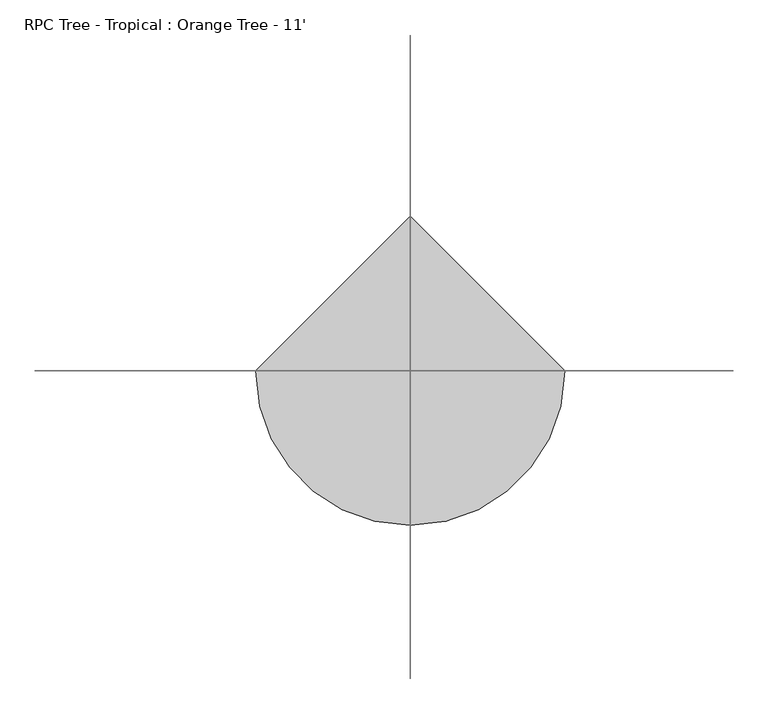
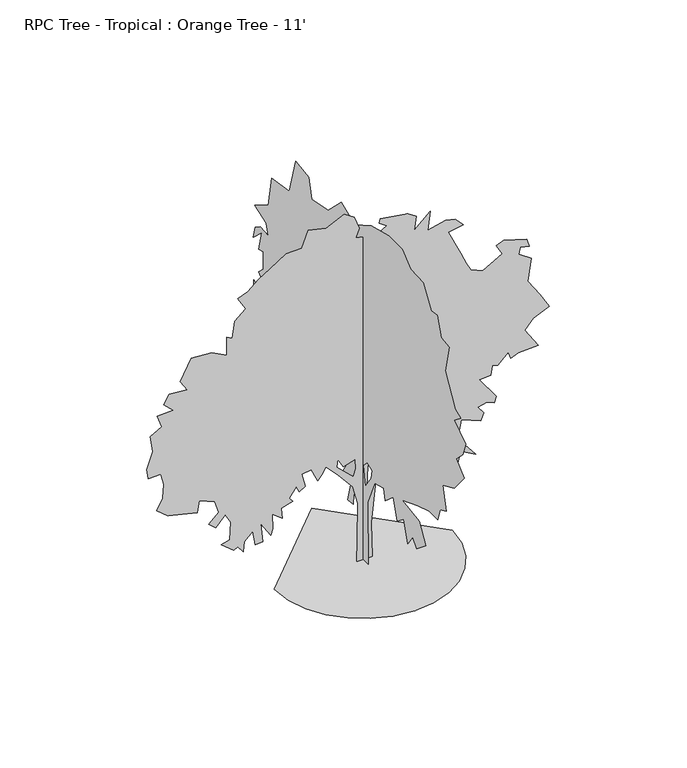
"""IFC4 building model written with IfcOpenShell, lengths in millimetres: geographic element geometry, RPC Tree - Tropical : Orange Tree - 11'."""

import ifcopenshell
import ifcopenshell.guid

model = None  # the IFC model being written
_history = None  # IfcOwnerHistory: only IFC2X3 demands one
_inside = {}  # id of a spatial element -> (the spatial element, [elements in it])
_under = {}  # id of a project, library or spatial element -> (it, [spatial elements below it])
_declared = {}  # id of a project -> (the project, [libraries it declares])
_typed = {}  # id of a type object -> (the type object, [elements of that type])
_made_of = {}  # id of a material, layer set ... -> (it, [elements and type objects made of it])


def new_model(schema):
    """Start an empty IFC model of exactly this schema.

    Asked for "IFC4X3", IfcOpenShell would pick the latest addendum, in which some entities
    have other attributes; the version numbers below select the first issue.
    IFC2X3 requires an IfcOwnerHistory on every rooted entity: one is made here for all.
    """
    global model, _history
    if schema == "IFC4X3":
        model = ifcopenshell.file(schema_version=(4, 3, 0, 0))
    else:
        model = ifcopenshell.file(schema=schema)
    _inside.clear()
    _under.clear()
    _declared.clear()
    _typed.clear()
    _made_of.clear()
    _history = None
    if model.schema == "IFC2X3":
        org = make("IfcOrganization", Name="unknown")
        user = make(
            "IfcPersonAndOrganization",
            ThePerson=make("IfcPerson", FamilyName="unknown"),
            TheOrganization=org,
        )
        app = make(
            "IfcApplication",
            ApplicationDeveloper=org,
            Version="unknown",
            ApplicationFullName="unknown",
            ApplicationIdentifier="unknown",
        )
        _history = make(
            "IfcOwnerHistory",
            OwningUser=user,
            OwningApplication=app,
            ChangeAction="ADDED",
            CreationDate=0,
        )
    return model


def make(cls, **values):
    """One entity of the class cls with the attributes given. An attribute that is None is left unset."""
    return model.create_entity(
        cls, **{name: value for name, value in values.items() if value is not None}
    )


def rooted(cls, **values):
    """An entity with a GlobalId (a new one), such as an element, a storey or a relation."""
    return make(cls, GlobalId=ifcopenshell.guid.new(), OwnerHistory=_history, **values)


def si_unit(unit_type, name, prefix=None):
    """IfcSIUnit, for example si_unit("LENGTHUNIT", "METRE", prefix="MILLI")."""
    return make("IfcSIUnit", UnitType=unit_type, Prefix=prefix, Name=name)


def assignment(units):
    """IfcUnitAssignment: the units of a project."""
    return None if units is None else make("IfcUnitAssignment", Units=units)


def point(xyz):
    """IfcCartesianPoint."""
    return None if xyz is None else make("IfcCartesianPoint", Coordinates=xyz)


def direction(xyz):
    """IfcDirection."""
    return None if xyz is None else make("IfcDirection", DirectionRatios=xyz)


def frame(location, z_axis=None, x_axis=None):
    """IfcAxis2Placement3D, a coordinate frame: its origin and axes. An axis left out is left unset."""
    return make(
        "IfcAxis2Placement3D",
        Location=point(location),
        Axis=direction(z_axis),
        RefDirection=direction(x_axis),
    )


def origin():
    """The frame at (0, 0, 0) with its axes left unset."""
    return frame((0.0, 0.0, 0.0))


def place(relative_to, where):
    """IfcLocalPlacement: puts the frame where relative to a parent placement (None: the world)."""
    return make(
        "IfcLocalPlacement", PlacementRelTo=relative_to, RelativePlacement=where
    )


def context(
    kind, dimensions, precision=None, world=None, true_north=None, identifier=None
):
    """IfcGeometricRepresentationContext, for example the 3D "Model" context."""
    return make(
        "IfcGeometricRepresentationContext",
        ContextIdentifier=identifier,
        ContextType=kind,
        CoordinateSpaceDimension=dimensions,
        Precision=precision,
        WorldCoordinateSystem=world,
        TrueNorth=true_north,
    )


def project(units=None, contexts=None):
    """IfcProject with its units and contexts."""
    return rooted(
        "IfcProject",
        Name="project",
        RepresentationContexts=contexts,
        UnitsInContext=assignment(units),
    )


def spatial(cls, under=None, at=None, **own):
    """A site, building, storey or space (cls), placed at a placement, below another one or the project."""
    s = rooted(cls, ObjectPlacement=at, **own)
    if under is not None:
        _under.setdefault(under.id(), (under, []))[1].append(s)
    return s


def point_list(points):
    """IfcCartesianPointList2D or 3D."""
    cls = (
        "IfcCartesianPointList2D" if len(points[0]) == 2 else "IfcCartesianPointList3D"
    )
    return make(cls, CoordList=points)


def triangles(points, corners, closed=None, point_numbers=None):
    """IfcTriangulatedFaceSet: each triangle names its three corners, points numbered from 1."""
    return make(
        "IfcTriangulatedFaceSet",
        Coordinates=point_list(points),
        Closed=closed,
        CoordIndex=corners,
        PnIndex=point_numbers,
    )


def shape(context_of_items, identifier, shape_type, items):
    """IfcShapeRepresentation: the items that make up one representation, for example the "Body"."""
    return make(
        "IfcShapeRepresentation",
        ContextOfItems=context_of_items,
        RepresentationIdentifier=identifier,
        RepresentationType=shape_type,
        Items=items,
    )


def source(mapping_origin, context_of_items, identifier, shape_type, items):
    """IfcRepresentationMap: a shape defined once, which mapped items show again and again."""
    return make(
        "IfcRepresentationMap",
        MappingOrigin=mapping_origin,
        MappedRepresentation=shape(context_of_items, identifier, shape_type, items),
    )


def transform(
    local_origin,
    x_axis=None,
    y_axis=None,
    z_axis=None,
    scale=None,
    scale2=None,
    scale3=None,
    uniform=True,
):
    """IfcCartesianTransformationOperator3D, or its non-uniform kind. x_axis, y_axis, z_axis: its Axis1, 2, 3."""
    if uniform:
        return make(
            "IfcCartesianTransformationOperator3D",
            Axis1=direction(x_axis),
            Axis2=direction(y_axis),
            LocalOrigin=point(local_origin),
            Scale=scale,
            Axis3=direction(z_axis),
        )
    return make(
        "IfcCartesianTransformationOperator3DnonUniform",
        Axis1=direction(x_axis),
        Axis2=direction(y_axis),
        LocalOrigin=point(local_origin),
        Scale=scale,
        Axis3=direction(z_axis),
        Scale2=scale2,
        Scale3=scale3,
    )


def mapped(mapping_source, mapping_target):
    """IfcMappedItem: shows the shape of a source again, moved by a transform."""
    return make(
        "IfcMappedItem", MappingSource=mapping_source, MappingTarget=mapping_target
    )


def made_of(thing, what):
    """Note that an element or type object is made of a material, layer set ...; save() writes the relation."""
    if what is not None:
        _made_of.setdefault(what.id(), (what, []))[1].append(thing)
    return thing


def element(
    cls,
    number,
    at=None,
    inside=None,
    cuts=None,
    type_object=None,
    material=None,
    context=None,
    identifier="Body",
    shape_type=None,
    held_by="IfcProductDefinitionShape",
    body=None,
    shapes=None,
    **own,
):
    """One element of the class cls, such as IfcWall. Its Tag is "e" and its number.

    at: its placement. inside: the storey or other place that contains it. cuts: it is an
    opening in that element (IfcRelVoidsElement). A single representation is given by context,
    identifier, shape_type and body (its items); several are given by shapes. held_by: the class
    of the entity that holds the representations. save() writes the other relations.
    """
    e = rooted(cls, Tag="e%d" % number, ObjectPlacement=at, **own)
    if body is not None:
        shapes = [shape(context, identifier, shape_type, body)]
    if shapes is not None:
        e.Representation = make(held_by, Representations=shapes)
    if inside is not None:
        _inside.setdefault(inside.id(), (inside, []))[1].append(e)
    if cuts is not None:
        rooted(
            "IfcRelVoidsElement", RelatingBuildingElement=cuts, RelatedOpeningElement=e
        )
    if type_object is not None:
        _typed.setdefault(type_object.id(), (type_object, []))[1].append(e)
    return made_of(e, material)


def aggregate(whole, parts):
    """IfcRelAggregates: a whole, such as a stair, and the parts it consists of."""
    return rooted("IfcRelAggregates", RelatingObject=whole, RelatedObjects=parts)


def save(model, path):
    """Write the relations noted so far, then the file.

    IfcRelAggregates (storeys below a building ...), IfcRelContainedInSpatialStructure (elements
    in a storey), IfcRelDefinesByType, IfcRelAssociatesMaterial and IfcRelDeclares: one each for
    every whole, place, type object, material and project.
    """
    for whole, parts in _under.values():
        aggregate(whole, parts)
    for where, things in _inside.values():
        rooted(
            "IfcRelContainedInSpatialStructure",
            RelatedElements=things,
            RelatingStructure=where,
        )
    for kind, things in _typed.values():
        rooted("IfcRelDefinesByType", RelatedObjects=things, RelatingType=kind)
    for what, things in _made_of.values():
        rooted("IfcRelAssociatesMaterial", RelatedObjects=things, RelatingMaterial=what)
    for by, libraries in _declared.values():
        rooted("IfcRelDeclares", RelatingContext=by, RelatedDefinitions=libraries)
    model.write(path)


def rpc_tree_tropical_orange_tree_11_d7a228f7(model_context):
    return source(origin(), model_context, "Body", "Tessellation", [
        triangles([(-803.9534712, 0.0, 6.05e-05), (-782.6987366, -184.2127929, 6.05e-05), (-722.1679836, -353.3826814, 6.05e-05), (-627.2075008, -502.663613, 6.05e-05), (-502.663613, -627.2075008, 6.05e-05), (-353.3826814, -722.1679836, 6.05e-05), (-184.2125386, -782.6987366, 6.05e-05), (3.51e-05, -803.9534712, 6.05e-05), (184.2127929, -782.6987366, 6.05e-05), (353.3826814, -722.1679836, 6.05e-05), (502.663613, -627.2075008, 6.05e-05), (627.2075008, -502.663613, 6.05e-05), (722.1679836, -353.3826814, 6.05e-05), (782.6987366, -184.2125386, 6.05e-05), (803.9534712, 7.03e-05, 6.05e-05), (-0.0001054, 803.9534712, 6.05e-05), (-4.73e-05, -77.0963933, 4.81e-05), (-2.95e-05, -72.7562921, 588.9525321), (-2.7e-05, -181.2628458, 836.3460434), (-3.2e-05, -320.1518609, 875.4087753), (-3.63e-05, -346.1919502, 771.2433311), (-3.87e-05, -472.0617019, 879.7495714), (-4.71e-05, -532.8235817, 688.7770712), (-4.92e-05, -632.6507006, 766.9024624), (-5.78e-05, -693.4151602, 571.5916368), (-5.81e-05, -775.878804, 684.4387459), (-6.3e-05, -832.3023949, 606.3134274), (-6.59e-05, -979.8713671, 727.8398031), (-5.62e-05, -875.7059229, 897.110503), (-4.32e-05, -610.9489002, 936.1731623), (-5.12e-05, -849.6633265, 1027.3185436), (-5.75e-05, -1031.9540892, 1088.0830032), (-6.35e-05, -1166.5029985, 1088.0830032), (-6.17e-05, -1201.224789, 1200.9301849), (-6.47e-05, -1296.7111118, 1244.3311695), (-5.59e-05, -1244.6283897, 1461.3462662), (-6.14e-05, -1422.5782837, 1543.8099827), (-6.28e-05, -1578.8289207, 1730.4416142), (-5.38e-05, -1452.9591328, 1843.2887959), (-5.55e-05, -1552.7863243, 1938.7749733), (-5.37e-05, -1600.5281776, 2068.9830139), (-4.21e-05, -1418.2374149, 2186.1685936), (-4.43e-05, -1526.7437279, 2272.9730335), (-3.95e-05, -1439.9391426, 2303.3564987), (-2.42e-05, -1279.3501076, 2576.8055054), (-1.94e-05, -1344.4529652, 2837.2061806), (-1.34e-05, -1218.5857206, 2850.2364899), (-5.3e-06, -1157.821261, 3028.1889999), (-1.5e-06, -1062.3375544, 3015.1586906), (9.7e-06, -940.8087078, 3206.14151), (1.89e-05, -741.1570135, 3214.8028999), (2.81e-05, -606.6080678, 3323.3116837), (3.75e-05, -398.2746723, 3327.6550232), (4.77e-05, -124.839264, 3258.2115875), (5.48e-05, 135.5766083, 3106.2941162), (6.66e-05, 339.5701524, 3197.4545403), (6.98e-05, 543.560172, 2997.8106216), (7.98e-05, 799.6379642, 2950.0585945), (8.73e-05, 847.3798176, 3128.0111046), (9.73e-05, 1051.3723806, 3158.3894829), (9.14e-05, 1151.1994995, 2811.1714325), (0.0001025, 1428.9739689, 2767.7627449), (9.64e-05, 1485.3975597, 2476.9656693), (0.0001018, 1689.3900501, 2351.0983521), (9.21e-05, 1515.7810249, 2285.9956398), (8.75e-05, 1481.0591618, 2186.1685936), (9.36e-05, 1606.926479, 2199.1910545), (9.54e-05, 1685.0517975, 2142.767609), (9.34e-05, 1715.4327919, 2029.9204273), (9.11e-05, 1580.8837372, 2155.7875992), (8.77e-05, 1632.9664593, 1964.815099), (8.51e-05, 1559.1820095, 1986.5168266), (8.02e-05, 1563.5228783, 1817.2460541), (8.14e-05, 1632.9664593, 1752.1433418), (7.34e-05, 1524.4602917, 1647.9754269), (7.38e-05, 1585.2246059, 1569.8525791), (8.13e-05, 1711.0919231, 1630.6144226), (7.79e-05, 1719.7736607, 1504.7472507), (7.16e-05, 1645.9890656, 1404.9226753), (7.48e-05, 1728.4527821, 1387.5618164), (7.27e-05, 1745.813641, 1292.0754936), (6.99e-05, 1650.3299343, 1339.817347), (6.11e-05, 1459.3574341, 1331.1382256), (6.23e-05, 1628.6282066, 1118.463925), (5.81e-05, 1520.1218937, 1140.1657253), (5.99e-05, 1611.2673477, 1062.0404068), (5.99e-05, 1698.0717876, 931.8322935), (5.77e-05, 1637.307328, 949.1932251), (5.11e-05, 1576.5454845, 818.9851845), (5.33e-05, 1572.2046158, 901.4513718), (4.88e-05, 1450.6756966, 931.8322935), (4.52e-05, 1402.9338432, 884.0904402), (4.47e-05, 1281.4075401, 1049.020344), (3.92e-05, 1264.0440651, 888.4313089), (3.71e-05, 1194.6004841, 923.1530994), (3.64e-05, 1116.4751656, 1018.6394222), (2.99e-05, 999.2896585, 975.2358215), (2.55e-05, 955.8861305, 892.7696342), (2.14e-05, 964.567868, 740.8623367), (1.6e-05, 873.4224867, 697.4588087), (1.6e-05, 916.8234713, 632.353553), (1.37e-05, 938.5251989, 523.8472401), (7.6e-06, 743.2143734, 610.6542961), (6.3e-06, 656.4073174, 697.4588087), (2.2e-06, 608.665464, 632.353553), (5.3e-06, 578.2845423, 779.9225252), (9e-07, 521.8609514, 719.1606091), (-7e-07, 456.7556594, 762.5615936), (1.1e-06, 465.4373606, 810.3059904), (-2e-06, 395.9937432, 810.3059904), (-7.3e-06, 335.22932, 723.5014778), (-6e-06, 291.8257738, 832.0077181), (-1e-05, 257.1039651, 749.5415308), (-1.02e-05, 317.8683884, 649.7169554), (-1.72e-05, 122.5560549, 710.4788715), (-1.74e-05, 192.000181, 597.6317262), (-2.03e-05, 244.0831574, 424.0226646), (-2.39e-05, 157.2781179, 432.7018224), (-2.16e-05, 144.2573102, 528.1880725), (-2.27e-05, 92.1740885, 571.5916368), (-2.48e-05, 44.4312178, 571.5916368), (-3.04e-05, 40.0908669, 389.3008378), (-4.11e-05, 61.7923765, 5.22e-05), (-2.23e-05, -137.8603261, 927.4914248), (-2.41e-05, -124.8395184, 849.3686497), (-2.39e-05, -33.6941257, 719.1606091), (-1.71e-05, -3.3121102, 901.4513718), (-1.8e-05, -64.07584, 962.2158314), (58.7260893, 2.69e-05, 920.6994701), (38.9260215, 3.03e-05, 877.8014345), (32.3258294, 4.22e-05, 683.1001648), (45.5259593, 4.5e-05, 626.9992287), (78.5256484, 3.59e-05, 755.7010386), (104.9259083, 2.72e-05, 881.1008698), (-56.7740963, 8.68e-05, 0.0), (-53.4738754, 7.45e-05, 204.6001204), (-50.1739042, 5.35e-05, 554.4008984), (-93.0740155, 4.51e-05, 726.0008165), (-225.0743068, 4.16e-05, 881.1008698), (-337.2739989, 3.93e-05, 1003.2012657), (-363.6747857, 4.36e-05, 950.3996922), (-409.8748363, 4.89e-05, 894.3012995), (-465.9733017, 4.39e-05, 1019.7011307), (-551.7745325, 4.85e-05, 1006.500701), (-522.0743105, 5.46e-05, 881.1008698), (-574.8733043, 5.89e-05, 848.1012125), (-604.5735263, 5.67e-05, 907.4991131), (-667.2734419, 6.47e-05, 818.4009905), (-634.2737846, 6.56e-05, 778.799774), (-739.8743156, 7.2e-05, 749.099552), (-729.9733938, 7.77e-05, 646.8010723), (-819.0740599, 7.74e-05, 716.0998947), (-815.7746246, 8.54e-05, 580.7991417), (-832.2744169, 8.94e-05, 524.7006763), (-924.6745909, 8.52e-05, 663.3008646), (-904.8752907, 9.48e-05, 488.3989677), (-970.8746778, 9.8e-05, 481.8000609), (-997.2754646, 9.11e-05, 617.1008503), (-1069.8737223, 9.86e-05, 544.4999765), (-1079.7746441, 0.0001046, 452.0998389), (-1129.2741663, 0.0001028, 518.0991898), (-1165.5758749, 0.0001058, 495.0004543), (-1281.0748569, 0.0001051, 590.7000635), (-1201.8750401, 0.0001005, 610.4993637), (-1195.2735535, 9.05e-05, 772.2009035), (-1241.4736404, 8.73e-05, 861.2990261), (-1327.2749439, 9.65e-05, 768.9013956), (-1389.9747505, 9.61e-05, 821.7004257), (-1300.8740845, 8.71e-05, 907.4991131), (-1337.1733223, 8.2e-05, 1019.7011307), (-1479.0755619, 8.49e-05, 1075.799596), (-1495.5752815, 9.19e-05, 970.2015358), (-1759.5754463, 9.97e-05, 1032.9014877), (-1858.5744907, 9.91e-05, 1115.4007399), (-1805.7755333, 9.07e-05, 1217.6992195), (-1799.1740467, 8.25e-05, 1349.70061), (-1825.5747608, 7.76e-05, 1451.999017), (-1937.7743076, 8.27e-05, 1448.6996544), (-1950.9746647, 7.78e-05, 1541.0998283), (-1894.8735832, 6.63e-05, 1692.9004463), (-1917.9749348, 5.84e-05, 1841.4015564), (-1815.6739117, 5.04e-05, 1900.7993843), (-1855.2749828, 4.52e-05, 2016.3009098), (-1713.3753593, 3.86e-05, 2022.8997803), (-1799.1740467, 3.75e-05, 2105.4015759), (-1746.3750893, 3.05e-05, 2184.6013927), (-1584.6734768, 2.4e-05, 2174.7003983), (-1650.6754074, 2.1e-05, 2273.6994427), (-1548.3743843, 5.5e-06, 2458.4999359), (-1366.8735443, -1.9e-06, 2448.6014122), (-1228.2732834, -3.6e-06, 2376.0006111), (-1228.2732834, -1.38e-05, 2547.5953697), (-1178.7737612, -1.44e-05, 2521.1995972), (-1158.974461, -2.45e-05, 2676.2973976), (-1056.6733652, -3.39e-05, 2758.7964317), (-1132.5736742, -3.79e-05, 2880.8942116), (-1040.1735003, -4.41e-05, 2917.1908333), (-941.1744558, -5.33e-05, 2999.6901581), (-835.5739248, -6.19e-05, 3065.7047333), (-693.6742287, -7.36e-05, 3158.1101395), (-555.0740041, -7.98e-05, 3161.4119728), (-495.6735237, -9.13e-05, 3309.9005836), (-333.9745637, -9.62e-05, 3273.6039619), (-172.2735144, -0.000108, 3352.8011627), (-79.8736311, -0.0001083, 3290.0884209), (-36.9737765, -0.0001029, 3167.990641), (-66.673751, -9.71e-05, 3092.0952736), (114.8263214, -0.0001024, 3049.1946945), (213.8264105, -0.0001101, 3105.303479), (144.5262982, -0.00011, 3154.8080154), (154.426457, -0.0001128, 3194.4067612), (401.9271747, -0.0001213, 3154.8080154), (477.8274837, -0.0001215, 3102.001355), (461.327655, -0.0001133, 2976.6014511), (606.5267864, -0.0001275, 3108.6053123), (580.126036, -0.0001159, 2933.700872), (745.1270473, -0.0001255, 2973.2996178), (827.6262268, -0.0001279, 2953.5130348), (900.2271006, -0.0001263, 2874.2902542), (768.2257828, -0.000119, 2847.8997139), (877.125749, -0.0001096, 2610.3081116), (929.9273226, -0.0001052, 2498.1010071), (969.525923, -0.0001024, 2422.2006981), (1078.4258892, -0.0001042, 2372.7011032), (1253.3278587, -0.000118, 2474.9995102), (1197.2268499, -0.0001212, 2570.7093658), (1266.525745, -0.000126, 2600.4020302), (1474.4272991, -0.0001312, 2534.4002449), (1497.5260345, -0.0001279, 2461.8017693), (1415.0268551, -0.0001252, 2478.3016342), (1401.826498, -0.0001211, 2418.9011902), (1514.0258995, -0.0001213, 2339.7013733), (1481.0261696, -0.0001075, 2131.7998192), (1593.2257164, -0.0001027, 1970.1008228), (1679.0268745, -9.78e-05, 1824.9016914), (1530.5257645, -8.76e-05, 1762.1992687), (1457.9274342, -7.91e-05, 1673.1010735), (1576.7258514, -7.35e-05, 1491.6002335), (1398.5269901, -6.51e-05, 1481.6993843), (1329.2255516, -6.03e-05, 1451.999017), (1309.4263241, -6.32e-05, 1514.701585), (1213.7267149, -5.39e-05, 1428.9002815), (1160.9276848, -5.24e-05, 1442.1006386), (1151.026763, -4.66e-05, 1352.9999725), (1045.426232, -4.18e-05, 1349.70061), (1197.2268499, -3.59e-05, 1138.4994753), (1180.726985, -3.16e-05, 1079.1015747), (1114.7275978, -3.05e-05, 1108.7992533), (1032.2258749, -2.57e-05, 1088.9999531), (1085.0273758, -2.39e-05, 1019.7011307), (1058.626589, -1.86e-05, 950.3996922), (883.7272356, -1.53e-05, 1023.0005659), (854.0270136, -3.8e-06, 851.4006477), (1012.4265747, 1.3e-06, 650.1005075), (877.125749, 2.7e-06, 726.0008165), (830.9257347, 1.63e-05, 531.2995831), (801.2255127, 1.04e-05, 653.3999428), (745.1270473, 8.7e-06, 722.7013813), (642.8259516, 1.59e-05, 676.5012943), (586.7274862, 2.47e-05, 570.900727), (487.725862, 2.15e-05, 696.3005945), (392.0262528, 1.76e-05, 831.6013475), (349.1256374, 2.48e-05, 742.5006815), (316.1259439, 1.76e-05, 887.6998129), (187.4264049, 2.7e-05, 824.999861), (114.8263214, 3.72e-05, 706.1989729), (71.9262193, 6.15e-05, 329.999443), (81.8261282, 8.08e-05, 0.0001067), (-178.8742198, 3.57e-05, 947.1002569), (-228.3742689, 3.25e-05, 1036.200923), (-238.2741733, 3.73e-05, 963.6001219), (-89.7740443, 3.95e-05, 818.4009905), (-66.6740053, 3.43e-05, 887.6998129), (-73.2739431, 2.91e-05, 980.0999868)], [[15, 16, 1], [14, 15, 1], [14, 1, 2], [13, 14, 2], [13, 2, 3], [13, 3, 4], [12, 13, 4], [11, 12, 4], [11, 4, 5], [11, 5, 6], [11, 6, 7], [11, 7, 8], [11, 8, 9], [11, 9, 10], [126, 17, 18], [88, 89, 90], [68, 69, 70], [67, 68, 70], [83, 84, 85], [86, 87, 88], [126, 18, 19], [125, 126, 19], [113, 114, 115], [104, 105, 106], [63, 64, 65], [80, 81, 82], [79, 80, 82], [66, 67, 70], [24, 25, 26], [101, 102, 103], [110, 111, 112], [42, 43, 44], [70, 71, 72], [20, 21, 22], [100, 101, 103], [116, 117, 118], [116, 118, 119], [76, 77, 78], [22, 23, 24], [93, 94, 95], [93, 95, 96], [76, 78, 79], [91, 92, 93], [45, 46, 47], [116, 119, 120], [115, 116, 120], [26, 27, 28], [26, 28, 29], [26, 29, 30], [24, 26, 30], [22, 24, 30], [123, 17, 126], [122, 123, 126], [121, 122, 126], [73, 74, 75], [79, 82, 83], [76, 79, 83], [37, 38, 39], [124, 125, 19], [59, 60, 61], [58, 59, 61], [106, 107, 108], [106, 108, 109], [66, 70, 72], [124, 19, 20], [34, 35, 36], [47, 48, 49], [100, 103, 104], [115, 120, 121], [115, 121, 126], [115, 126, 127], [40, 41, 42], [39, 40, 42], [32, 33, 34], [113, 115, 127], [112, 113, 127], [61, 62, 63], [55, 56, 57], [98, 99, 100], [98, 100, 104], [98, 104, 106], [86, 88, 90], [86, 90, 91], [85, 86, 91], [85, 91, 93], [83, 85, 93], [75, 76, 83], [36, 37, 39], [49, 50, 51], [83, 93, 96], [32, 34, 36], [97, 98, 106], [31, 32, 36], [42, 44, 45], [97, 106, 109], [51, 52, 53], [75, 83, 96], [75, 96, 97], [61, 63, 65], [61, 65, 66], [58, 61, 66], [57, 58, 66], [75, 97, 109], [73, 75, 109], [72, 73, 109], [66, 72, 109], [57, 66, 109], [57, 109, 110], [57, 110, 112], [57, 112, 127], [57, 127, 128], [55, 57, 128], [54, 55, 128], [53, 54, 128], [51, 53, 128], [49, 51, 128], [47, 49, 128], [45, 47, 128], [42, 45, 128], [39, 42, 128], [36, 39, 128], [31, 36, 128], [30, 31, 128], [30, 128, 124], [30, 124, 20], [30, 20, 22], [135, 130, 131], [130, 135, 136], [130, 136, 137], [135, 131, 132], [253, 254, 255], [255, 256, 257], [130, 137, 138], [272, 129, 130], [272, 130, 138], [129, 272, 273], [262, 263, 264], [214, 215, 216], [272, 138, 139], [271, 272, 139], [271, 139, 140], [159, 160, 161], [150, 151, 152], [153, 154, 155], [152, 153, 155], [162, 163, 164], [218, 219, 220], [237, 238, 239], [228, 229, 230], [227, 228, 230], [191, 192, 193], [141, 142, 143], [148, 149, 150], [259, 260, 261], [182, 183, 184], [217, 218, 220], [161, 162, 164], [270, 271, 140], [129, 273, 274], [195, 196, 197], [268, 135, 132], [267, 268, 132], [266, 267, 132], [266, 132, 133], [265, 266, 133], [265, 133, 134], [246, 247, 248], [245, 246, 248], [234, 235, 236], [140, 141, 143], [225, 226, 227], [225, 227, 230], [225, 230, 231], [167, 168, 169], [166, 167, 169], [239, 240, 241], [145, 146, 147], [144, 145, 147], [255, 257, 258], [253, 255, 258], [171, 172, 173], [237, 239, 241], [216, 217, 220], [245, 248, 249], [250, 251, 252], [249, 250, 252], [155, 156, 157], [155, 157, 158], [210, 211, 212], [209, 210, 212], [177, 178, 179], [243, 244, 245], [201, 202, 203], [184, 185, 186], [184, 186, 187], [274, 269, 270], [173, 174, 175], [171, 173, 175], [159, 161, 164], [177, 179, 180], [158, 159, 164], [158, 164, 165], [155, 158, 165], [171, 175, 176], [180, 181, 182], [188, 189, 190], [187, 188, 190], [187, 190, 191], [231, 232, 233], [245, 249, 252], [212, 213, 214], [209, 212, 214], [203, 204, 205], [203, 205, 206], [203, 206, 207], [201, 203, 207], [264, 265, 134], [208, 209, 214], [241, 242, 243], [225, 231, 233], [224, 225, 233], [233, 234, 236], [224, 233, 236], [224, 236, 237], [224, 237, 241], [224, 241, 243], [223, 224, 243], [223, 243, 245], [152, 155, 165], [152, 165, 166], [259, 261, 262], [258, 259, 262], [253, 258, 262], [252, 253, 262], [252, 262, 264], [245, 252, 264], [223, 245, 264], [223, 264, 134], [223, 134, 129], [223, 129, 274], [223, 274, 270], [222, 223, 270], [221, 222, 270], [220, 221, 270], [216, 220, 270], [214, 216, 270], [208, 214, 270], [207, 208, 270], [201, 207, 270], [200, 201, 270], [199, 200, 270], [198, 199, 270], [197, 198, 270], [195, 197, 270], [194, 195, 270], [193, 194, 270], [191, 193, 270], [191, 270, 140], [191, 140, 143], [191, 143, 144], [187, 191, 144], [184, 187, 144], [182, 184, 144], [180, 182, 144], [177, 180, 144], [176, 177, 144], [171, 176, 144], [170, 171, 144], [170, 144, 147], [169, 170, 147], [166, 169, 147], [152, 166, 147], [152, 147, 148], [152, 148, 150]], closed=False),
    ])


if __name__ == "__main__":
    model = new_model("IFC4")
    model_context = context("Model", 3, world=origin())
    ifc_project = project(units=[si_unit("LENGTHUNIT", "METRE", prefix="MILLI")], contexts=[model_context])
    site = spatial("IfcSite", under=ifc_project)
    building = spatial("IfcBuilding", under=site)
    placement = place(None, origin())
    rpc_tree_tropical_orange_tree_11_shape = rpc_tree_tropical_orange_tree_11_d7a228f7(model_context)
    element("IfcGeographicElement", 1, ObjectType="RPC Tree - Tropical : Orange Tree - 11'", at=placement, inside=building, context=model_context, shape_type="MappedRepresentation", body=[
        mapped(rpc_tree_tropical_orange_tree_11_shape, transform((0.0, 0.0, 0.0), x_axis=(1.0, 0.0, 0.0), y_axis=(0.0, 1.0, 0.0), z_axis=(0.0, 0.0, 1.0))),
    ])
    save(model, "model.ifc")

# Revit data of these elements
# Type "RPC Tree - Tropical : Orange Tree - 11'"
#   built-in parameter 1005198 = "{2, 15},{39, RPC-16-FVGW-4XXX-7J75-W000-ST1L-LVER-AU},{1, 0},{1, 0},{2, 35},{1, 8},{5, Color},{1, 0},{1, 0},{3, 0.8},{3, 0.8},{3, 0.8},{1, 8},{7, BBoxMin},{1, 0},{1, 0},{1, 0},{1, 0},{1, 0},{1, 8},{7, BBoxMax},{1, 0},{1, 0},{1, 0},{1, 0},{1, 0},{2, 11},{9, RPCTypeId},{1, 0},{1, 0},{39, RPC-16-FVGW-4XXX-7J75-W000-ST1L-LVER-AU},{1, 6},{14, RPCPlantHeight},{1, 0},{1, 0},{2, 11},{2, 11},{7, keyword},{1, 0},{1, 0},{77, :Geometry:RPC:Orange Tree:citrus sinensis:valencia:orange:tropical:tree:fruit},{2, 11},{8, category},{1, 0},{1, 0},{17, :Trees [Tropical]},{2, 11},{12, LocalizedUID},{1, 0},{1, 0},{11, Orange Tree},{2, 14},{6, Height},{1, 0},{1, 0},{2, 11},{1, 2},{16, Cast Reflections},{1, 0},{1, 0},{1, 0},{1, 2},{12, Cast Shadows},{1, 0},{1, 0},{1, 1},{1, 2},{9, Lock View},{1, 0},{1, 0},{1, 0},{1, 4},{5, ViewC},{1, 0},{1, 0},{1, 0},{2, 11},{20, AdvancedUIDefinition},{1, 0},{1, 0},{0, },{2, 11},{10, AssetLibID},{1, 0},{1, 0},{36, 4D3F6E72-3F99-4203-98E9-AF80B3C7A7A4},{2, 11},{10, BaseSchema},{1, 0},{1, 0},{9, RPCSchema},{2, 11},{12, ExchangeGUID},{1, 0},{1, 0},{0, },{1, 2},{6, Hidden},{1, 0},{1, 0},{1, 0},{1, 4},{11, RPCCategory},{1, 0},{1, 0},{1, 0},{2, 11},{8, RPCImage},{1, 0},{1, 0},{0, },{1, 4},{13, SchemaVersion},{1, 0},{1, 0},{1, 4},{2, 11},{12, UIDefinition},{1, 0},{1, 0},{0, },{2, 11},{6, UIName},{1, 0},{1, 0},{39, RPC-16-FVGW-4XXX-7J75-W000-ST1L-LVER-AU},{2, 11},{11, VersionGUID},{1, 0},{1, 0},{9, RPCSchema},{2, 11},{9, assettype},{1, 0},{1, 0},{11, RPCGeometry},{2, 11},{11, description},{1, 0},{1, 0},{0, },{2, 11},{9, localname},{1, 0},{1, 0},{3, RPC},{2, 11},{9, localtype},{1, 0},{1, 0},{3, RPC},{1, 4},{8, revision},{1, 0},{1, 0},{1, 1},{2, 11},{9, thumbnail},{1, 0},{1, 0},{0, },{1, 4},{7, version},{1, 0},{1, 0},{1, 1},{1, 2},{20, RPC_Cast Reflections},{1, 0},{1, 0},{1, 1},{1, 2},{16, RPC_Cast Shadows},{1, 0},{1, 0},{1, 1},{1, 2},{13, RPC_Lock View},{1, 0},{1, 0},{1, 0},{1, 4},{9, RPC_ViewC},{1, 0},{1, 0},{1, 0},{21, assetlibrary_base.fbx},{1, 5},"
#   built-in parameter 1005195 = "RPC-16-FVGW-4XXX-7J75-W000-ST1L-LVER-AU"
#   Type Comments = "Orange Tree"
#   Assembly Code = "G2050500"
#   Height = 11' - 0"
#   Plan Symbol = element 763022
#   Default Elevation = 0
